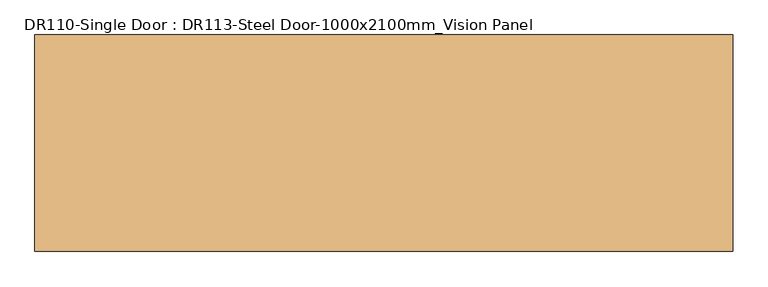
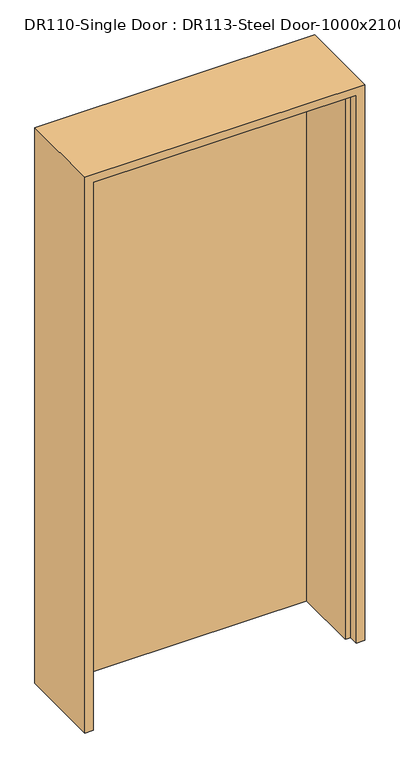
"""IFC4 building model written with IfcOpenShell, lengths in millimetres: door geometry, DR110-Single Door : DR113-Steel Door-1000x2100mm_Vision Panel."""

from ifc_helpers import new_model, si_unit, origin, origin_with_axes, place, context, project, spatial, polyline, outline, extrude, faceted_brep, source, transform, mapped, element, save


def dr110_single_door_dr113_steel_door_1000x2100mm_vision_panel_15eccd39(model_context):
    return source(origin(), model_context, "Body", "SolidModel", [
        extrude(outline(polyline([(470.0, 155.0), (470.0, 120.0), (-470.0, 120.0), (-470.0, 155.0), (470.0, 155.0)])), origin_with_axes(), (0.0, 0.0, 1.0), 2070.0),
        faceted_brep([(470.0, 155.0, 0.0), (500.0, 155.0, 0.0), (500.0, -155.0, 0.0), (470.0, -155.0, 0.0), (470.0, -120.0, 0.0), (450.0, -120.0, 0.0), (450.0, 120.0, 0.0), (470.0, 120.0, 0.0), (470.0, 155.0, 2070.0), (-470.0, 155.0, 2070.0), (-470.0, 155.0, 0.0), (-500.0, 155.0, 0.0), (-500.0, 155.0, 2100.0), (500.0, 155.0, 2100.0), (500.0, -155.0, 2100.0), (-500.0, -155.0, 2100.0), (-500.0, -155.0, 0.0), (-470.0, -155.0, 0.0), (-470.0, -155.0, 2070.0), (470.0, -155.0, 2070.0), (470.0, -120.0, 2070.0), (-470.0, -120.0, 2070.0), (-470.0, -120.0, 0.0), (-450.0, -120.0, 0.0), (-450.0, -120.0, 2050.0), (450.0, -120.0, 2050.0), (450.0, 120.0, 2050.0), (-450.0, 120.0, 2050.0), (-450.0, 120.0, 0.0), (-470.0, 120.0, 0.0), (-470.0, 120.0, 2070.0), (470.0, 120.0, 2070.0)], [[[0, 1, 2, 3, 4, 5, 6, 7]], [[1, 0, 8, 9, 10, 11, 12, 13]], [[2, 1, 13, 14]], [[3, 2, 14, 15, 16, 17, 18, 19]], [[4, 3, 19, 20]], [[5, 4, 20, 21, 22, 23, 24, 25]], [[6, 5, 25, 26]], [[7, 6, 26, 27, 28, 29, 30, 31]], [[0, 7, 31, 8]], [[9, 30, 29, 10]], [[10, 29, 28, 23, 22, 17, 16, 11]], [[15, 12, 11, 16]], [[21, 18, 17, 22]], [[27, 24, 23, 28]], [[14, 13, 12, 15]], [[20, 19, 18, 21]], [[26, 25, 24, 27]], [[8, 31, 30, 9]]]),
    ])


if __name__ == "__main__":
    model = new_model("IFC4")
    model_context = context("Model", 3, world=origin())
    ifc_project = project(units=[si_unit("LENGTHUNIT", "METRE", prefix="MILLI")], contexts=[model_context])
    site = spatial("IfcSite", under=ifc_project)
    building = spatial("IfcBuilding", under=site)
    placement = place(None, origin())
    dr110_single_door_dr113_steel_door_1000x2100mm_vision_panel_shape = dr110_single_door_dr113_steel_door_1000x2100mm_vision_panel_15eccd39(model_context)
    element("IfcDoor", 1, ObjectType="DR110-Single Door : DR113-Steel Door-1000x2100mm_Vision Panel", at=placement, inside=building, context=model_context, shape_type="MappedRepresentation", body=[
        mapped(dr110_single_door_dr113_steel_door_1000x2100mm_vision_panel_shape, transform((0.0, 0.0, 0.0), x_axis=(1.0, 0.0, 0.0), y_axis=(0.0, 1.0, 0.0), z_axis=(0.0, 0.0, 1.0))),
    ])
    save(model, "model.ifc")

# Revit data of these elements
# Type "DR110-Single Door : DR113-Steel Door-1000x2100mm_Vision Panel"
#   Type Mark = "SD"
#   Analytic Construction = "<None>"
#   프레임 투영 외부. = 25 mm
#   프레임 투영 내부. = 25 mm
#   프레임 폭 = 75 mm
#   Height = 2100 mm
#   Width = 1000 mm
#   Define Thermal Properties by = 1
#   문 패널 = SD1 문 패널
#   문 프레임 = A04AQ098-00002_Steel Door_non FP_single
#   Function = (empty or 0)
#   Wall Closure = (empty or 0)
# Element 1 (IfcDoor, "DR110-Single Door : DR113-Steel Door-1000x2100mm_Vision Panel")
#   Materials on its faces: "A04AQ098-00002_Steel Door_non FP_single", "SD1 문 패널"
# Materials
#   "SD1 문 패널": class "금속", colour RGB 247 247 247, transparency 0, Description = "STEEL DOOR (1000Wx2100H)"
#   "A04AQ098-00002_Steel Door_non FP_single": class "금속", colour RGB 247 247 247, transparency 0, Description = "Steel Door", W00) Work Master Code = "A04AQ098-00002", W01) Work Master_Lv1 = "Finishing Work", W02) Work Master_Lv2 = "Door & Window Work", W03) Work Master_Spec.1 = "Steel Door w/ Steel Frame", W04) Work Master_Spec.2 = "Fire Protective Rating: N/A, Single Door", W05) Work Master_Spec.3 = "w/ Hardware & Accessories", Cost = 0
